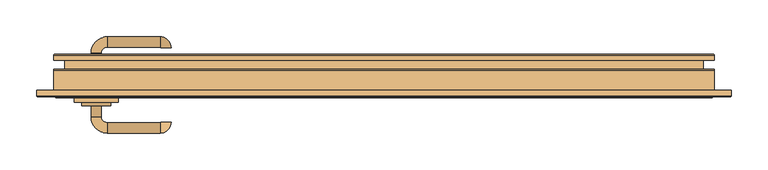
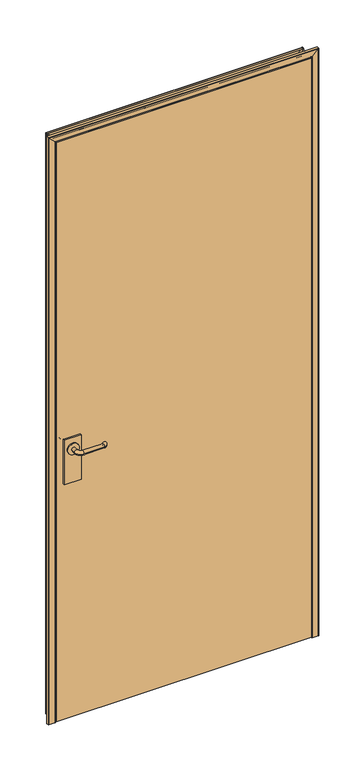
"""IFC4 building model written with IfcOpenShell, lengths in millimetres: door geometry, Porta Simples de Abrir : 90x210cm - Aduela Metálica de Canto."""

from ifc_helpers import new_model, si_unit, point, frame, frame_2d, origin, place, context, project, spatial, polyline, circle_curve, ellipse_curve, trimmed, segment, composite_curve, outline, extrude, source, transform, mapped, element, save
from ifc_brep_helpers import plane_surface, cylinder_surface, revolved_surface, advanced_brep


def door_e47fb599(model_context):
    return source(origin(), model_context, "Body", "SolidModel", [
        extrude(outline(composite_curve([segment(trimmed(circle_curve(frame_2d((1050.0, -392.0)), 20.0), [point((1050.0, -412.0))], [point((1050.0, -372.0))], False, "CARTESIAN"), True, "CONTINUOUS"), segment(trimmed(circle_curve(frame_2d((1050.0, -392.0)), 20.0), [point((1050.0, -372.0))], [point((1050.0, -412.0))], False, "CARTESIAN"), True, "CONTINUOUS")], self_intersect=False)), frame((0.0, -54.6, 0.0), z_axis=(0.0, 1.0, 0.0), x_axis=(0.0, 0.0, 1.0)), (0.0, 0.0, 1.0), 4.5929895),
        advanced_brep(
        [(-385.0, -50.0070105, 1050.0), (-399.0, -50.0070105, 1050.0), (-385.0, -34.6, 1050.0), (-399.0, -34.6, 1050.0), (-377.0, -12.6, 1050.0), (-377.0, -26.6, 1050.0), (-305.0, -26.6, 1050.0), (-305.0, -12.6, 1050.0), (-304.0, -27.6, 1050.0), (-290.0, -27.6, 1050.0)],
        [
            (0, 1, circle_curve(frame((-392.0, -50.0070105, 1050.0), z_axis=(0.0, -1.0, 0.0), x_axis=(-1.0, 0.0, 0.0)), 7.0)),
            (1, 0, circle_curve(frame((-392.0, -50.0070105, 1050.0), z_axis=(0.0, -1.0, 0.0), x_axis=(-1.0, 0.0, 0.0)), 7.0)),
            (0, 2),
            (2, 3, circle_curve(frame((-392.0, -34.6, 1050.0), z_axis=(0.0, -1.0, 0.0), x_axis=(-1.0, 0.0, 0.0)), 7.0)),
            (3, 1),
            (3, 2, circle_curve(frame((-392.0, -34.6, 1050.0), z_axis=(0.0, -1.0, 0.0), x_axis=(-1.0, 0.0, 0.0)), 7.0)),
            (4, 3, circle_curve(frame((-377.0, -34.6, 1050.0), z_axis=(0.0, 0.0, 1.0), x_axis=(-1.0, 0.0, 0.0)), 22.0)),
            (2, 5, circle_curve(frame((-377.0, -34.6, 1050.0), z_axis=(0.0, 0.0, -1.0), x_axis=(-1.0, 0.0, 0.0)), 8.0)),
            (5, 4, circle_curve(frame((-377.0, -19.6, 1050.0), z_axis=(-1.0, 0.0, 0.0), x_axis=(0.0, 1.0, 0.0)), 7.0)),
            (4, 5, circle_curve(frame((-377.0, -19.6, 1050.0), z_axis=(-1.0, 0.0, 0.0), x_axis=(0.0, 1.0, 0.0)), 7.0)),
            (5, 6),
            (6, 7, circle_curve(frame((-305.0, -19.6, 1050.0), z_axis=(-1.0, 0.0, 0.0), x_axis=(0.0, 1.0, 0.0)), 7.0)),
            (7, 4),
            (7, 6, circle_curve(frame((-305.0, -19.6, 1050.0), z_axis=(-1.0, 0.0, 0.0), x_axis=(0.0, 1.0, 0.0)), 7.0)),
            (8, 9, circle_curve(frame((-297.0, -27.6, 1050.0), z_axis=(0.0, -1.0, 0.0), x_axis=(1.0, 0.0, 0.0)), 7.0)),
            (9, 8, circle_curve(frame((-297.0, -27.6, 1050.0), z_axis=(0.0, -1.0, 0.0), x_axis=(1.0, 0.0, 0.0)), 7.0)),
            (9, 7, circle_curve(frame((-305.0, -27.6, 1050.0), z_axis=(0.0, 0.0, 1.0), x_axis=(0.0, 1.0, 0.0)), 15.0)),
            (6, 8, circle_curve(frame((-305.0, -27.6, 1050.0), z_axis=(0.0, 0.0, -1.0), x_axis=(0.0, 1.0, 0.0)), 1.0)),
        ],
        [
            plane_surface(frame((-392.0, -50.0070105, 1050.0), z_axis=(0.0, -1.0, 0.0), x_axis=(0.0, 0.0, 1.0))),
            cylinder_surface(frame((-392.0, -50.0070105, 1050.0), z_axis=(0.0, -1.0, 0.0), x_axis=(-1.0, 0.0, 0.0)), 7.0),
            revolved_surface(trimmed(ellipse_curve(frame((-392.0, -34.6, 1050.0), z_axis=(0.0, -1.0, 0.0), x_axis=(-1.0, 0.0, 0.0)), 7.0, 7.0), [point((-385.0, -34.6, 1050.0))], [point((-399.0, -34.6, 1050.0))], True, "CARTESIAN"), (-377.0, -34.6, 1050.0), (0.0, 0.0, -1.0)),
            revolved_surface(trimmed(ellipse_curve(frame((-392.0, -34.6, 1050.0), z_axis=(0.0, -1.0, 0.0), x_axis=(-1.0, 0.0, 0.0)), 7.0, 7.0), [point((-399.0, -34.6, 1050.0))], [point((-385.0, -34.6, 1050.0))], True, "CARTESIAN"), (-377.0, -34.6, 1050.0), (0.0, 0.0, -1.0)),
            cylinder_surface(frame((-377.0, -19.6, 1050.0), z_axis=(-1.0, 0.0, 0.0), x_axis=(0.0, 1.0, 0.0)), 7.0),
            plane_surface(frame((-297.0, -27.6, 1050.0), z_axis=(0.0, -1.0, 0.0), x_axis=(0.0, 0.0, 1.0))),
            revolved_surface(trimmed(ellipse_curve(frame((-305.0, -19.6, 1050.0), z_axis=(-1.0, 0.0, 0.0), x_axis=(0.0, 1.0, 0.0)), 7.0, 7.0), [point((-305.0, -26.6, 1050.0))], [point((-305.0, -12.6, 1050.0))], True, "CARTESIAN"), (-305.0, -27.6, 1050.0), (0.0, 0.0, -1.0)),
            revolved_surface(trimmed(ellipse_curve(frame((-305.0, -19.6, 1050.0), z_axis=(-1.0, 0.0, 0.0), x_axis=(0.0, 1.0, 0.0)), 7.0, 7.0), [point((-305.0, -12.6, 1050.0))], [point((-305.0, -26.6, 1050.0))], True, "CARTESIAN"), (-305.0, -27.6, 1050.0), (0.0, 0.0, -1.0)),
        ],
        [
            (0, [[1, 2]]),
            (1, [[-1, 3, 4, 5]]),
            (1, [[-2, -5, 6, -3]]),
            (2, [[7, -4, 8, 9]]),
            (3, [[-8, -6, -7, 10]]),
            (4, [[-9, 11, 12, 13]]),
            (4, [[-10, -13, 14, -11]]),
            (5, [[15, 16]]),
            (6, [[17, -12, 18, -16]]),
            (7, [[-18, -14, -17, -15]]),
        ],
    ),
        extrude(outline(polyline([(-362.0, -60.6), (-422.0, -60.6), (-422.0, -54.6), (-362.0, -54.6), (-362.0, -60.6)])), frame((0.0, 0.0, 925.0), z_axis=(0.0, 0.0, 1.0), x_axis=(1.0, 0.0, 0.0)), (0.0, 0.0, 1.0), 165.0),
        extrude(outline(composite_curve([segment(trimmed(circle_curve(frame_2d((1050.0, -392.0)), 20.0), [point((1050.0, -412.0))], [point((1050.0, -372.0))], False, "CARTESIAN"), True, "CONTINUOUS"), segment(trimmed(circle_curve(frame_2d((1050.0, -392.0)), 20.0), [point((1050.0, -372.0))], [point((1050.0, -412.0))], False, "CARTESIAN"), True, "CONTINUOUS")], self_intersect=False)), frame((0.0, -106.1929895, 0.0), z_axis=(0.0, 1.0, 0.0), x_axis=(0.0, 0.0, 1.0)), (0.0, 0.0, 1.0), 4.5929895),
        advanced_brep(
        [(-385.0, -106.1929895, 1050.0), (-399.0, -106.1929895, 1050.0), (-399.0, -121.6, 1050.0), (-385.0, -121.6, 1050.0), (-377.0, -143.6, 1050.0), (-377.0, -129.6, 1050.0), (-305.0, -143.6, 1050.0), (-305.0, -129.6, 1050.0), (-304.0, -128.6, 1050.0), (-290.0, -128.6, 1050.0)],
        [
            (0, 1, circle_curve(frame((-392.0, -106.1929895, 1050.0), z_axis=(0.0, 1.0, 0.0), x_axis=(-1.0, 0.0, 0.0)), 7.0)),
            (1, 0, circle_curve(frame((-392.0, -106.1929895, 1050.0), z_axis=(0.0, 1.0, 0.0), x_axis=(-1.0, 0.0, 0.0)), 7.0)),
            (1, 2),
            (2, 3, circle_curve(frame((-392.0, -121.6, 1050.0), z_axis=(0.0, 1.0, 0.0), x_axis=(-1.0, 0.0, 0.0)), 7.0)),
            (3, 0),
            (3, 2, circle_curve(frame((-392.0, -121.6, 1050.0), z_axis=(0.0, 1.0, 0.0), x_axis=(-1.0, 0.0, 0.0)), 7.0)),
            (4, 5, circle_curve(frame((-377.0, -136.6, 1050.0), z_axis=(-1.0, 0.0, 0.0), x_axis=(0.0, -1.0, 0.0)), 7.0)),
            (5, 3, circle_curve(frame((-377.0, -121.6, 1050.0), z_axis=(0.0, 0.0, -1.0), x_axis=(-1.0, 0.0, 0.0)), 8.0)),
            (2, 4, circle_curve(frame((-377.0, -121.6, 1050.0), z_axis=(0.0, 0.0, 1.0), x_axis=(-1.0, 0.0, 0.0)), 22.0)),
            (5, 4, circle_curve(frame((-377.0, -136.6, 1050.0), z_axis=(-1.0, 0.0, 0.0), x_axis=(0.0, -1.0, 0.0)), 7.0)),
            (4, 6),
            (6, 7, circle_curve(frame((-305.0, -136.6, 1050.0), z_axis=(-1.0, 0.0, 0.0), x_axis=(0.0, -1.0, 0.0)), 7.0)),
            (7, 5),
            (7, 6, circle_curve(frame((-305.0, -136.6, 1050.0), z_axis=(-1.0, 0.0, 0.0), x_axis=(0.0, -1.0, 0.0)), 7.0)),
            (8, 9, circle_curve(frame((-297.0, -128.6, 1050.0), z_axis=(0.0, 1.0, 0.0), x_axis=(1.0, 0.0, 0.0)), 7.0)),
            (9, 8, circle_curve(frame((-297.0, -128.6, 1050.0), z_axis=(0.0, 1.0, 0.0), x_axis=(1.0, 0.0, 0.0)), 7.0)),
            (8, 7, circle_curve(frame((-305.0, -128.6, 1050.0), z_axis=(0.0, 0.0, -1.0), x_axis=(0.0, -1.0, 0.0)), 1.0)),
            (6, 9, circle_curve(frame((-305.0, -128.6, 1050.0), z_axis=(0.0, 0.0, 1.0), x_axis=(0.0, -1.0, 0.0)), 15.0)),
        ],
        [
            plane_surface(frame((-392.0, -106.1929895, 1050.0), z_axis=(0.0, 1.0, 0.0), x_axis=(0.0, 0.0, 1.0))),
            cylinder_surface(frame((-392.0, -106.1929895, 1050.0), z_axis=(0.0, 1.0, 0.0), x_axis=(-1.0, 0.0, 0.0)), 7.0),
            revolved_surface(trimmed(ellipse_curve(frame((-392.0, -121.6, 1050.0), z_axis=(0.0, -1.0, 0.0), x_axis=(-1.0, 0.0, 0.0)), 7.0, 7.0), [point((-385.0, -121.6, 1050.0))], [point((-399.0, -121.6, 1050.0))], True, "CARTESIAN"), (-377.0, -121.6, 1050.0), (0.0, 0.0, -1.0)),
            revolved_surface(trimmed(ellipse_curve(frame((-392.0, -121.6, 1050.0), z_axis=(0.0, -1.0, 0.0), x_axis=(-1.0, 0.0, 0.0)), 7.0, 7.0), [point((-399.0, -121.6, 1050.0))], [point((-385.0, -121.6, 1050.0))], True, "CARTESIAN"), (-377.0, -121.6, 1050.0), (0.0, 0.0, -1.0)),
            cylinder_surface(frame((-377.0, -136.6, 1050.0), z_axis=(-1.0, 0.0, 0.0), x_axis=(0.0, -1.0, 0.0)), 7.0),
            plane_surface(frame((-297.0, -128.6, 1050.0), z_axis=(0.0, 1.0, 0.0), x_axis=(0.0, 0.0, 1.0))),
            revolved_surface(trimmed(ellipse_curve(frame((-305.0, -136.6, 1050.0), z_axis=(1.0, 0.0, 0.0), x_axis=(0.0, -1.0, 0.0)), 7.0, 7.0), [point((-305.0, -129.6, 1050.0))], [point((-305.0, -143.6, 1050.0))], True, "CARTESIAN"), (-305.0, -128.6, 1050.0), (0.0, 0.0, -1.0)),
            revolved_surface(trimmed(ellipse_curve(frame((-305.0, -136.6, 1050.0), z_axis=(1.0, 0.0, 0.0), x_axis=(0.0, -1.0, 0.0)), 7.0, 7.0), [point((-305.0, -143.6, 1050.0))], [point((-305.0, -129.6, 1050.0))], True, "CARTESIAN"), (-305.0, -128.6, 1050.0), (0.0, 0.0, -1.0)),
        ],
        [
            (0, [[1, 2]]),
            (1, [[3, 4, 5, -2]]),
            (1, [[-5, 6, -3, -1]]),
            (2, [[7, 8, -4, 9]]),
            (3, [[10, -9, -6, -8]]),
            (4, [[11, 12, 13, -7]]),
            (4, [[-13, 14, -11, -10]]),
            (5, [[15, 16]]),
            (6, [[-15, 17, -12, 18]]),
            (7, [[-16, -18, -14, -17]]),
        ],
    ),
        extrude(outline(polyline([(-362.0, -95.6), (-362.0, -101.6), (-422.0, -101.6), (-422.0, -95.6), (-362.0, -95.6)])), frame((0.0, 0.0, 925.0), z_axis=(0.0, 0.0, 1.0), x_axis=(1.0, 0.0, 0.0)), (0.0, 0.0, 1.0), 165.0),
        extrude(outline(polyline([(447.0, -60.6), (447.0, -95.6), (-447.0, -95.6), (-447.0, -60.6), (447.0, -60.6)])), frame((0.0, 0.0, 53.0), z_axis=(0.0, 0.0, 1.0), x_axis=(1.0, 0.0, 0.0)), (0.0, 0.0, 1.0), 2143.0),
        advanced_brep(
        [(-435.5, -36.6, 50.0), (-434.0, -38.1, 50.0), (-434.0, -56.1, 50.0), (-435.5, -57.6, 50.0), (-448.55, -57.6, 50.0), (-449.05, -58.1, 50.0), (-449.05, -93.1, 50.0), (-450.55, -94.6, 50.0), (-471.55, -94.6, 50.0), (-473.05, -93.1, 50.0), (-473.05, -85.6, 50.0), (-472.05, -85.6, 50.0), (-472.05, -93.1, 50.0), (-471.55, -93.6, 50.0), (-450.55, -93.6, 50.0), (-450.05, -93.1, 50.0), (-450.05, -58.1, 50.0), (-448.55, -56.6, 50.0), (-435.5, -56.6, 50.0), (-435.0, -56.1, 50.0), (-435.0, -38.1, 50.0), (-435.5, -37.6, 50.0), (-448.5, -37.6, 50.0), (-449.0, -38.1, 50.0), (-449.0, -44.6, 50.0), (-450.0, -44.6, 50.0), (-450.0, -38.1, 50.0), (-448.5, -36.6, 50.0), (-448.5, -36.6, 2198.5), (-435.5, -36.6, 2185.5), (-450.0, -38.1, 2200.0), (-450.0, -44.6, 2200.0), (-449.0, -44.6, 2199.0), (-449.0, -38.1, 2199.0), (-448.5, -37.6, 2198.5), (-435.5, -37.6, 2185.5), (-435.0, -38.1, 2185.0), (-435.0, -56.1, 2185.0), (-435.5, -56.6, 2185.5), (-448.55, -56.6, 2198.55), (-450.05, -58.1, 2200.05), (-450.05, -93.1, 2200.05), (-450.55, -93.6, 2200.55), (-471.55, -93.6, 2221.55), (-472.05, -93.1, 2222.05), (-472.05, -85.6, 2222.05), (-473.05, -85.6, 2223.05), (-473.05, -93.1, 2223.05), (-471.55, -94.6, 2221.55), (-450.55, -94.6, 2200.55), (-449.05, -93.1, 2199.05), (-449.05, -58.1, 2199.05), (-448.55, -57.6, 2198.55), (-435.5, -57.6, 2185.5), (-434.0, -56.1, 2184.0), (-434.0, -38.1, 2184.0), (435.5, -36.6, 50.0), (448.5, -36.6, 50.0), (450.0, -38.1, 50.0), (450.0, -44.6, 50.0), (449.0, -44.6, 50.0), (449.0, -38.1, 50.0), (448.5, -37.6, 50.0), (435.5, -37.6, 50.0), (435.0, -38.1, 50.0), (435.0, -56.1, 50.0), (435.5, -56.6, 50.0), (448.55, -56.6, 50.0), (450.05, -58.1, 50.0), (450.05, -93.1, 50.0), (450.55, -93.6, 50.0), (471.55, -93.6, 50.0), (472.05, -93.1, 50.0), (472.05, -85.6, 50.0), (473.05, -85.6, 50.0), (473.05, -93.1, 50.0), (471.55, -94.6, 50.0), (450.55, -94.6, 50.0), (449.05, -93.1, 50.0), (449.05, -58.1, 50.0), (448.55, -57.6, 50.0), (435.5, -57.6, 50.0), (434.0, -56.1, 50.0), (434.0, -38.1, 50.0), (435.5, -36.6, 2185.5), (434.0, -38.1, 2184.0), (434.0, -56.1, 2184.0), (435.5, -57.6, 2185.5), (448.55, -57.6, 2198.55), (449.05, -58.1, 2199.05), (449.05, -93.1, 2199.05), (450.55, -94.6, 2200.55), (471.55, -94.6, 2221.55), (473.05, -93.1, 2223.05), (473.05, -85.6, 2223.05), (472.05, -85.6, 2222.05), (472.05, -93.1, 2222.05), (471.55, -93.6, 2221.55), (450.55, -93.6, 2200.55), (450.05, -93.1, 2200.05), (450.05, -58.1, 2200.05), (448.55, -56.6, 2198.55), (435.5, -56.6, 2185.5), (435.0, -56.1, 2185.0), (435.0, -38.1, 2185.0), (435.5, -37.6, 2185.5), (448.5, -37.6, 2198.5), (449.0, -38.1, 2199.0), (449.0, -44.6, 2199.0), (450.0, -44.6, 2200.0), (450.0, -38.1, 2200.0), (448.5, -36.6, 2198.5)],
        [
            (0, 1, circle_curve(frame((-435.5, -38.1, 50.0), z_axis=(0.0, 0.0, -1.0), x_axis=(1.0, 0.0, 0.0)), 1.5)),
            (1, 2),
            (2, 3, circle_curve(frame((-435.5, -56.1, 50.0), z_axis=(0.0, 0.0, -1.0), x_axis=(1.0, 0.0, 0.0)), 1.5)),
            (3, 4),
            (4, 5, circle_curve(frame((-448.55, -58.1, 50.0), z_axis=(0.0, 0.0, 1.0), x_axis=(1.0, 0.0, 0.0)), 0.5)),
            (5, 6),
            (6, 7, circle_curve(frame((-450.55, -93.1, 50.0), z_axis=(0.0, 0.0, -1.0), x_axis=(1.0, 0.0, 0.0)), 1.5)),
            (7, 8),
            (8, 9, circle_curve(frame((-471.55, -93.1, 50.0), z_axis=(0.0, 0.0, -1.0), x_axis=(1.0, 0.0, 0.0)), 1.5)),
            (9, 10),
            (10, 11),
            (11, 12),
            (12, 13, circle_curve(frame((-471.55, -93.1, 50.0), z_axis=(0.0, 0.0, 1.0), x_axis=(1.0, 0.0, 0.0)), 0.5)),
            (13, 14),
            (14, 15, circle_curve(frame((-450.55, -93.1, 50.0), z_axis=(0.0, 0.0, 1.0), x_axis=(1.0, 0.0, 0.0)), 0.5)),
            (15, 16),
            (16, 17, circle_curve(frame((-448.55, -58.1, 50.0), z_axis=(0.0, 0.0, -1.0), x_axis=(1.0, 0.0, 0.0)), 1.5)),
            (17, 18),
            (18, 19, circle_curve(frame((-435.5, -56.1, 50.0), z_axis=(0.0, 0.0, 1.0), x_axis=(1.0, 0.0, 0.0)), 0.5)),
            (19, 20),
            (20, 21, circle_curve(frame((-435.5, -38.1, 50.0), z_axis=(0.0, 0.0, 1.0), x_axis=(1.0, 0.0, 0.0)), 0.5)),
            (21, 22),
            (22, 23, circle_curve(frame((-448.5, -38.1, 50.0), z_axis=(0.0, 0.0, 1.0), x_axis=(1.0, 0.0, 0.0)), 0.5)),
            (23, 24),
            (24, 25),
            (25, 26),
            (26, 27, circle_curve(frame((-448.5, -38.1, 50.0), z_axis=(0.0, 0.0, -1.0), x_axis=(1.0, 0.0, 0.0)), 1.5)),
            (27, 0),
            (27, 28),
            (28, 29),
            (29, 0),
            (26, 30),
            (30, 28, ellipse_curve(frame((-448.5, -38.1, 2198.5), z_axis=(-0.7071067811865475, 0.0, -0.7071067811865475), x_axis=(0.7071067811865474, 0.0, -0.7071067811865476)), 2.1213203, 1.5)),
            (25, 31),
            (31, 30),
            (24, 32),
            (32, 31),
            (23, 33),
            (33, 32),
            (22, 34),
            (34, 33, ellipse_curve(frame((-448.5, -38.1, 2198.5), z_axis=(0.7071067811865475, 0.0, 0.7071067811865475), x_axis=(-0.7071067811865474, 0.0, 0.7071067811865476)), 0.7071068, 0.5)),
            (21, 35),
            (35, 34),
            (20, 36),
            (36, 35, ellipse_curve(frame((-435.5, -38.1, 2185.5), z_axis=(0.7071067811865475, 0.0, 0.7071067811865475), x_axis=(-0.7071067811865474, 0.0, 0.7071067811865476)), 0.7071068, 0.5)),
            (19, 37),
            (37, 36),
            (18, 38),
            (38, 37, ellipse_curve(frame((-435.5, -56.1, 2185.5), z_axis=(0.7071067811865475, 0.0, 0.7071067811865475), x_axis=(-0.7071067811865474, 0.0, 0.7071067811865476)), 0.7071068, 0.5)),
            (17, 39),
            (39, 38),
            (16, 40),
            (40, 39, ellipse_curve(frame((-448.55, -58.1, 2198.55), z_axis=(-0.7071067811865475, 0.0, -0.7071067811865475), x_axis=(0.7071067811865474, 0.0, -0.7071067811865476)), 2.1213203, 1.5)),
            (15, 41),
            (41, 40),
            (14, 42),
            (42, 41, ellipse_curve(frame((-450.55, -93.1, 2200.55), z_axis=(0.7071067811865475, 0.0, 0.7071067811865475), x_axis=(-0.7071067811865474, 0.0, 0.7071067811865476)), 0.7071068, 0.5)),
            (13, 43),
            (43, 42),
            (12, 44),
            (44, 43, ellipse_curve(frame((-471.55, -93.1, 2221.55), z_axis=(0.7071067811865475, 0.0, 0.7071067811865475), x_axis=(-0.7071067811865474, 0.0, 0.7071067811865476)), 0.7071068, 0.5)),
            (11, 45),
            (45, 44),
            (10, 46),
            (46, 45),
            (9, 47),
            (47, 46),
            (8, 48),
            (48, 47, ellipse_curve(frame((-471.55, -93.1, 2221.55), z_axis=(-0.7071067811865475, 0.0, -0.7071067811865475), x_axis=(0.7071067811865474, 0.0, -0.7071067811865476)), 2.1213203, 1.5)),
            (7, 49),
            (49, 48),
            (6, 50),
            (50, 49, ellipse_curve(frame((-450.55, -93.1, 2200.55), z_axis=(-0.7071067811865475, 0.0, -0.7071067811865475), x_axis=(0.7071067811865474, 0.0, -0.7071067811865476)), 2.1213203, 1.5)),
            (5, 51),
            (51, 50),
            (4, 52),
            (52, 51, ellipse_curve(frame((-448.55, -58.1, 2198.55), z_axis=(0.7071067811865475, 0.0, 0.7071067811865475), x_axis=(-0.7071067811865474, 0.0, 0.7071067811865476)), 0.7071068, 0.5)),
            (3, 53),
            (53, 52),
            (2, 54),
            (54, 53, ellipse_curve(frame((-435.5, -56.1, 2185.5), z_axis=(-0.7071067811865475, 0.0, -0.7071067811865475), x_axis=(0.7071067811865474, 0.0, -0.7071067811865476)), 2.1213203, 1.5)),
            (1, 55),
            (55, 54),
            (29, 55, ellipse_curve(frame((-435.5, -38.1, 2185.5), z_axis=(-0.7071067811865475, 0.0, -0.7071067811865475), x_axis=(0.7071067811865474, 0.0, -0.7071067811865476)), 2.1213203, 1.5)),
            (56, 57),
            (57, 58, circle_curve(frame((448.5, -38.1, 50.0), z_axis=(0.0, 0.0, -1.0), x_axis=(-1.0, 0.0, 0.0)), 1.5)),
            (58, 59),
            (59, 60),
            (60, 61),
            (61, 62, circle_curve(frame((448.5, -38.1, 50.0), z_axis=(0.0, 0.0, 1.0), x_axis=(-1.0, 0.0, 0.0)), 0.5)),
            (62, 63),
            (63, 64, circle_curve(frame((435.5, -38.1, 50.0), z_axis=(0.0, 0.0, 1.0), x_axis=(-1.0, 0.0, 0.0)), 0.5)),
            (64, 65),
            (65, 66, circle_curve(frame((435.5, -56.1, 50.0), z_axis=(0.0, 0.0, 1.0), x_axis=(-1.0, 0.0, 0.0)), 0.5)),
            (66, 67),
            (67, 68, circle_curve(frame((448.55, -58.1, 50.0), z_axis=(0.0, 0.0, -1.0), x_axis=(-1.0, 0.0, 0.0)), 1.5)),
            (68, 69),
            (69, 70, circle_curve(frame((450.55, -93.1, 50.0), z_axis=(0.0, 0.0, 1.0), x_axis=(-1.0, 0.0, 0.0)), 0.5)),
            (70, 71),
            (71, 72, circle_curve(frame((471.55, -93.1, 50.0), z_axis=(0.0, 0.0, 1.0), x_axis=(-1.0, 0.0, 0.0)), 0.5)),
            (72, 73),
            (73, 74),
            (74, 75),
            (75, 76, circle_curve(frame((471.55, -93.1, 50.0), z_axis=(0.0, 0.0, -1.0), x_axis=(-1.0, 0.0, 0.0)), 1.5)),
            (76, 77),
            (77, 78, circle_curve(frame((450.55, -93.1, 50.0), z_axis=(0.0, 0.0, -1.0), x_axis=(-1.0, 0.0, 0.0)), 1.5)),
            (78, 79),
            (79, 80, circle_curve(frame((448.55, -58.1, 50.0), z_axis=(0.0, 0.0, 1.0), x_axis=(-1.0, 0.0, 0.0)), 0.5)),
            (80, 81),
            (81, 82, circle_curve(frame((435.5, -56.1, 50.0), z_axis=(0.0, 0.0, -1.0), x_axis=(-1.0, 0.0, 0.0)), 1.5)),
            (82, 83),
            (83, 56, circle_curve(frame((435.5, -38.1, 50.0), z_axis=(0.0, 0.0, -1.0), x_axis=(-1.0, 0.0, 0.0)), 1.5)),
            (84, 56),
            (83, 85),
            (85, 84, ellipse_curve(frame((435.5, -38.1, 2185.5), z_axis=(0.7071067811865475, 0.0, -0.7071067811865475), x_axis=(0.7071067811865474, 0.0, 0.7071067811865476)), 2.1213203, 1.5)),
            (82, 86),
            (86, 85),
            (81, 87),
            (87, 86, ellipse_curve(frame((435.5, -56.1, 2185.5), z_axis=(0.7071067811865475, 0.0, -0.7071067811865475), x_axis=(0.7071067811865474, 0.0, 0.7071067811865476)), 2.1213203, 1.5)),
            (80, 88),
            (88, 87),
            (79, 89),
            (89, 88, ellipse_curve(frame((448.55, -58.1, 2198.55), z_axis=(-0.7071067811865475, 0.0, 0.7071067811865475), x_axis=(-0.7071067811865474, 0.0, -0.7071067811865476)), 0.7071068, 0.5)),
            (78, 90),
            (90, 89),
            (77, 91),
            (91, 90, ellipse_curve(frame((450.55, -93.1, 2200.55), z_axis=(0.7071067811865475, 0.0, -0.7071067811865475), x_axis=(0.7071067811865474, 0.0, 0.7071067811865476)), 2.1213203, 1.5)),
            (76, 92),
            (92, 91),
            (75, 93),
            (93, 92, ellipse_curve(frame((471.55, -93.1, 2221.55), z_axis=(0.7071067811865475, 0.0, -0.7071067811865475), x_axis=(0.7071067811865474, 0.0, 0.7071067811865476)), 2.1213203, 1.5)),
            (74, 94),
            (94, 93),
            (73, 95),
            (95, 94),
            (72, 96),
            (96, 95),
            (71, 97),
            (97, 96, ellipse_curve(frame((471.55, -93.1, 2221.55), z_axis=(-0.7071067811865475, 0.0, 0.7071067811865475), x_axis=(-0.7071067811865474, 0.0, -0.7071067811865476)), 0.7071068, 0.5)),
            (70, 98),
            (98, 97),
            (69, 99),
            (99, 98, ellipse_curve(frame((450.55, -93.1, 2200.55), z_axis=(-0.7071067811865475, 0.0, 0.7071067811865475), x_axis=(-0.7071067811865474, 0.0, -0.7071067811865476)), 0.7071068, 0.5)),
            (68, 100),
            (100, 99),
            (67, 101),
            (101, 100, ellipse_curve(frame((448.55, -58.1, 2198.55), z_axis=(0.7071067811865475, 0.0, -0.7071067811865475), x_axis=(0.7071067811865474, 0.0, 0.7071067811865476)), 2.1213203, 1.5)),
            (66, 102),
            (102, 101),
            (65, 103),
            (103, 102, ellipse_curve(frame((435.5, -56.1, 2185.5), z_axis=(-0.7071067811865475, 0.0, 0.7071067811865475), x_axis=(-0.7071067811865474, 0.0, -0.7071067811865476)), 0.7071068, 0.5)),
            (64, 104),
            (104, 103),
            (63, 105),
            (105, 104, ellipse_curve(frame((435.5, -38.1, 2185.5), z_axis=(-0.7071067811865475, 0.0, 0.7071067811865475), x_axis=(-0.7071067811865474, 0.0, -0.7071067811865476)), 0.7071068, 0.5)),
            (62, 106),
            (106, 105),
            (61, 107),
            (107, 106, ellipse_curve(frame((448.5, -38.1, 2198.5), z_axis=(-0.7071067811865475, 0.0, 0.7071067811865475), x_axis=(-0.7071067811865474, 0.0, -0.7071067811865476)), 0.7071068, 0.5)),
            (60, 108),
            (108, 107),
            (59, 109),
            (109, 108),
            (58, 110),
            (110, 109),
            (57, 111),
            (111, 110, ellipse_curve(frame((448.5, -38.1, 2198.5), z_axis=(0.7071067811865475, 0.0, -0.7071067811865475), x_axis=(0.7071067811865474, 0.0, 0.7071067811865476)), 2.1213203, 1.5)),
            (84, 111),
            (28, 111),
            (84, 29),
            (30, 110),
            (31, 109),
            (32, 108),
            (33, 107),
            (34, 106),
            (35, 105),
            (36, 104),
            (37, 103),
            (38, 102),
            (39, 101),
            (40, 100),
            (41, 99),
            (42, 98),
            (43, 97),
            (44, 96),
            (45, 95),
            (46, 94),
            (47, 93),
            (48, 92),
            (49, 91),
            (50, 90),
            (51, 89),
            (52, 88),
            (53, 87),
            (54, 86),
            (55, 85),
        ],
        [
            plane_surface(frame((-450.0, -34.4996086, 50.0), z_axis=(0.0, 0.0, -1.0), x_axis=(1.0, 0.0, 0.0))),
            plane_surface(frame((-435.5, -36.6, 50.0), z_axis=(0.0, 1.0, 0.0), x_axis=(0.0, 0.0, 1.0))),
            cylinder_surface(frame((-448.5, -38.1, 50.0), z_axis=(0.0, 0.0, -1.0), x_axis=(1.0, 0.0, 0.0)), 1.5),
            plane_surface(frame((-450.0, -38.1, 50.0), z_axis=(-1.0, 0.0, 0.0), x_axis=(0.0, 0.0, 1.0))),
            plane_surface(frame((-450.0, -44.6, 50.0), z_axis=(0.0, -1.0, 0.0), x_axis=(0.0, 0.0, 1.0))),
            plane_surface(frame((-449.0, -44.6, 50.0), z_axis=(1.0, 0.0, 0.0), x_axis=(0.0, 0.0, 1.0))),
            revolved_surface(polyline([(-448.0, -38.1, 2199.000000013303), (-448.0, -38.1, 50.0)]), (-448.5, -38.1, 50.0), (0.0, 0.0, 1.0)),
            plane_surface(frame((-448.5, -37.6, 50.0), z_axis=(0.0, -1.0, 0.0), x_axis=(0.0, 0.0, 1.0))),
            revolved_surface(polyline([(-435.0, -38.1, 2186.000000013303), (-435.0, -38.1, 50.0)]), (-435.5, -38.1, 50.0), (0.0, 0.0, 1.0)),
            plane_surface(frame((-435.0, -38.1, 50.0), z_axis=(-1.0, 0.0, 0.0), x_axis=(0.0, 0.0, 1.0))),
            revolved_surface(polyline([(-435.0, -56.1, 2186.000000013303), (-435.0, -56.1, 50.0)]), (-435.5, -56.1, 50.0), (0.0, 0.0, 1.0)),
            plane_surface(frame((-435.5, -56.6, 50.0), z_axis=(0.0, 1.0, 0.0), x_axis=(0.0, 0.0, 1.0))),
            cylinder_surface(frame((-448.55, -58.1, 50.0), z_axis=(0.0, 0.0, -1.0), x_axis=(1.0, 0.0, 0.0)), 1.5),
            plane_surface(frame((-450.05, -58.1, 50.0), z_axis=(-1.0, 0.0, 0.0), x_axis=(0.0, 0.0, 1.0))),
            revolved_surface(polyline([(-450.05, -93.1, 2201.0500000133034), (-450.05, -93.1, 50.0)]), (-450.55, -93.1, 50.0), (0.0, 0.0, 1.0)),
            plane_surface(frame((-450.55, -93.6, 50.0), z_axis=(0.0, 1.0, 0.0), x_axis=(0.0, 0.0, 1.0))),
            revolved_surface(polyline([(-471.05, -93.1, 2222.0500000133034), (-471.05, -93.1, 50.0)]), (-471.55, -93.1, 50.0), (0.0, 0.0, 1.0)),
            plane_surface(frame((-472.05, -93.1, 50.0), z_axis=(1.0, 0.0, 0.0), x_axis=(0.0, 0.0, 1.0))),
            plane_surface(frame((-472.05, -85.6, 50.0), z_axis=(0.0, 1.0, 0.0), x_axis=(0.0, 0.0, 1.0))),
            plane_surface(frame((-473.05, -85.6, 50.0), z_axis=(-1.0, 0.0, 0.0), x_axis=(0.0, 0.0, 1.0))),
            cylinder_surface(frame((-471.55, -93.1, 50.0), z_axis=(0.0, 0.0, -1.0), x_axis=(1.0, 0.0, 0.0)), 1.5),
            plane_surface(frame((-471.55, -94.6, 50.0), z_axis=(0.0, -1.0, 0.0), x_axis=(0.0, 0.0, 1.0))),
            cylinder_surface(frame((-450.55, -93.1, 50.0), z_axis=(0.0, 0.0, -1.0), x_axis=(1.0, 0.0, 0.0)), 1.5),
            plane_surface(frame((-449.05, -93.1, 50.0), z_axis=(1.0, 0.0, 0.0), x_axis=(0.0, 0.0, 1.0))),
            revolved_surface(polyline([(-448.05, -58.1, 2199.0500000133034), (-448.05, -58.1, 50.0)]), (-448.55, -58.1, 50.0), (0.0, 0.0, 1.0)),
            plane_surface(frame((-448.55, -57.6, 50.0), z_axis=(0.0, -1.0, 0.0), x_axis=(0.0, 0.0, 1.0))),
            cylinder_surface(frame((-435.5, -56.1, 50.0), z_axis=(0.0, 0.0, -1.0), x_axis=(1.0, 0.0, 0.0)), 1.5),
            plane_surface(frame((-434.0, -56.1, 50.0), z_axis=(1.0, 0.0, 0.0), x_axis=(0.0, 0.0, 1.0))),
            cylinder_surface(frame((-435.5, -38.1, 50.0), z_axis=(0.0, 0.0, -1.0), x_axis=(1.0, 0.0, 0.0)), 1.5),
            plane_surface(frame((450.0, -34.4996086, 50.0), z_axis=(0.0, 0.0, -1.0), x_axis=(-1.0, 0.0, 0.0))),
            cylinder_surface(frame((435.5, -38.1, 2200.0), z_axis=(0.0, 0.0, 1.0), x_axis=(-1.0, 0.0, 0.0)), 1.5),
            plane_surface(frame((434.0, -56.1, 2184.0), z_axis=(-1.0, 0.0, 0.0), x_axis=(0.0, 0.0, -1.0))),
            cylinder_surface(frame((435.5, -56.1, 2200.0), z_axis=(0.0, 0.0, 1.0), x_axis=(-1.0, 0.0, 0.0)), 1.5),
            plane_surface(frame((448.55, -57.6, 2198.55), z_axis=(0.0, -1.0, 0.0), x_axis=(0.0, 0.0, -1.0))),
            revolved_surface(polyline([(448.05, -58.1, 50.0), (448.05, -58.1, 2199.0500000133034)]), (448.55, -58.1, 2200.0), (0.0, 0.0, -1.0)),
            plane_surface(frame((449.05, -93.1, 2199.05), z_axis=(-1.0, 0.0, 0.0), x_axis=(0.0, 0.0, -1.0))),
            cylinder_surface(frame((450.55, -93.1, 2200.0), z_axis=(0.0, 0.0, 1.0), x_axis=(-1.0, 0.0, 0.0)), 1.5),
            plane_surface(frame((471.55, -94.6, 2221.55), z_axis=(0.0, -1.0, 0.0), x_axis=(0.0, 0.0, -1.0))),
            cylinder_surface(frame((471.55, -93.1, 2200.0), z_axis=(0.0, 0.0, 1.0), x_axis=(-1.0, 0.0, 0.0)), 1.5),
            plane_surface(frame((473.05, -85.6, 2223.05), z_axis=(1.0, 0.0, 0.0), x_axis=(0.0, 0.0, -1.0))),
            plane_surface(frame((472.05, -85.6, 2222.05), z_axis=(0.0, 1.0, 0.0), x_axis=(0.0, 0.0, -1.0))),
            plane_surface(frame((472.05, -93.1, 2222.05), z_axis=(-1.0, 0.0, 0.0), x_axis=(0.0, 0.0, -1.0))),
            revolved_surface(polyline([(471.05, -93.1, 50.0), (471.05, -93.1, 2222.0500000133034)]), (471.55, -93.1, 2200.0), (0.0, 0.0, -1.0)),
            plane_surface(frame((450.55, -93.6, 2200.55), z_axis=(0.0, 1.0, 0.0), x_axis=(0.0, 0.0, -1.0))),
            revolved_surface(polyline([(450.05, -93.1, 50.0), (450.05, -93.1, 2201.0500000133034)]), (450.55, -93.1, 2200.0), (0.0, 0.0, -1.0)),
            plane_surface(frame((450.05, -58.1, 2200.05), z_axis=(1.0, 0.0, 0.0), x_axis=(0.0, 0.0, -1.0))),
            cylinder_surface(frame((448.55, -58.1, 2200.0), z_axis=(0.0, 0.0, 1.0), x_axis=(-1.0, 0.0, 0.0)), 1.5),
            plane_surface(frame((435.5, -56.6, 2185.5), z_axis=(0.0, 1.0, 0.0), x_axis=(0.0, 0.0, -1.0))),
            revolved_surface(polyline([(435.0, -56.1, 50.0), (435.0, -56.1, 2186.000000013303)]), (435.5, -56.1, 2200.0), (0.0, 0.0, -1.0)),
            plane_surface(frame((435.0, -38.1, 2185.0), z_axis=(1.0, 0.0, 0.0), x_axis=(0.0, 0.0, -1.0))),
            revolved_surface(polyline([(435.0, -38.1, 50.0), (435.0, -38.1, 2186.000000013303)]), (435.5, -38.1, 2200.0), (0.0, 0.0, -1.0)),
            plane_surface(frame((448.5, -37.6, 2198.5), z_axis=(0.0, -1.0, 0.0), x_axis=(0.0, 0.0, -1.0))),
            revolved_surface(polyline([(448.0, -38.1, 50.0), (448.0, -38.1, 2199.000000013303)]), (448.5, -38.1, 2200.0), (0.0, 0.0, -1.0)),
            plane_surface(frame((449.0, -44.6, 2199.0), z_axis=(-1.0, 0.0, 0.0), x_axis=(0.0, 0.0, -1.0))),
            plane_surface(frame((450.0, -44.6, 2200.0), z_axis=(0.0, -1.0, 0.0), x_axis=(0.0, 0.0, -1.0))),
            plane_surface(frame((450.0, -38.1, 2200.0), z_axis=(1.0, 0.0, 0.0), x_axis=(0.0, 0.0, -1.0))),
            cylinder_surface(frame((448.5, -38.1, 2200.0), z_axis=(0.0, 0.0, 1.0), x_axis=(-1.0, 0.0, 0.0)), 1.5),
            plane_surface(frame((435.5, -36.6, 2185.5), z_axis=(0.0, 1.0, 0.0), x_axis=(0.0, 0.0, -1.0))),
            plane_surface(frame((-435.5, -36.6, 2185.5), z_axis=(0.0, 1.0, 0.0), x_axis=(1.0, 0.0, 0.0))),
            cylinder_surface(frame((-450.0, -38.1, 2198.5), z_axis=(-1.0, 0.0, 0.0), x_axis=(0.0, 0.0, -1.0)), 1.5),
            plane_surface(frame((-450.0, -38.1, 2200.0), z_axis=(0.0, 0.0, 1.0), x_axis=(1.0, 0.0, 0.0))),
            plane_surface(frame((-450.0, -44.6, 2200.0), z_axis=(0.0, -1.0, 0.0), x_axis=(1.0, 0.0, 0.0))),
            plane_surface(frame((-449.0, -44.6, 2199.0), z_axis=(0.0, 0.0, -1.0), x_axis=(1.0, 0.0, 0.0))),
            revolved_surface(polyline([(449.00000001330307, -38.1, 2198.0), (-449.0000000133031, -38.1, 2198.0)]), (-450.0, -38.1, 2198.5), (1.0, 0.0, 0.0)),
            plane_surface(frame((-448.5, -37.6, 2198.5), z_axis=(0.0, -1.0, 0.0), x_axis=(1.0, 0.0, 0.0))),
            revolved_surface(polyline([(436.00000001330307, -38.1, 2185.0), (-436.0000000133031, -38.1, 2185.0)]), (-450.0, -38.1, 2185.5), (1.0, 0.0, 0.0)),
            plane_surface(frame((-435.0, -38.1, 2185.0), z_axis=(0.0, 0.0, 1.0), x_axis=(1.0, 0.0, 0.0))),
            revolved_surface(polyline([(436.00000001330307, -56.1, 2185.0), (-436.0000000133031, -56.1, 2185.0)]), (-450.0, -56.1, 2185.5), (1.0, 0.0, 0.0)),
            plane_surface(frame((-435.5, -56.6, 2185.5), z_axis=(0.0, 1.0, 0.0), x_axis=(1.0, 0.0, 0.0))),
            cylinder_surface(frame((-450.0, -58.1, 2198.55), z_axis=(-1.0, 0.0, 0.0), x_axis=(0.0, 0.0, -1.0)), 1.5),
            plane_surface(frame((-450.05, -58.1, 2200.05), z_axis=(0.0, 0.0, 1.0), x_axis=(1.0, 0.0, 0.0))),
            revolved_surface(polyline([(451.050000013303, -93.1, 2200.05), (-451.05000001330313, -93.1, 2200.05)]), (-450.0, -93.1, 2200.55), (1.0, 0.0, 0.0)),
            plane_surface(frame((-450.55, -93.6, 2200.55), z_axis=(0.0, 1.0, 0.0), x_axis=(1.0, 0.0, 0.0))),
            revolved_surface(polyline([(472.050000013303, -93.1, 2221.05), (-472.05000001330313, -93.1, 2221.05)]), (-450.0, -93.1, 2221.55), (1.0, 0.0, 0.0)),
            plane_surface(frame((-472.05, -93.1, 2222.05), z_axis=(0.0, 0.0, -1.0), x_axis=(1.0, 0.0, 0.0))),
            plane_surface(frame((-472.05, -85.6, 2222.05), z_axis=(0.0, 1.0, 0.0), x_axis=(1.0, 0.0, 0.0))),
            plane_surface(frame((-473.05, -85.6, 2223.05), z_axis=(0.0, 0.0, 1.0), x_axis=(1.0, 0.0, 0.0))),
            cylinder_surface(frame((-450.0, -93.1, 2221.55), z_axis=(-1.0, 0.0, 0.0), x_axis=(0.0, 0.0, -1.0)), 1.5),
            plane_surface(frame((-471.55, -94.6, 2221.55), z_axis=(0.0, -1.0, 0.0), x_axis=(1.0, 0.0, 0.0))),
            cylinder_surface(frame((-450.0, -93.1, 2200.55), z_axis=(-1.0, 0.0, 0.0), x_axis=(0.0, 0.0, -1.0)), 1.5),
            plane_surface(frame((-449.05, -93.1, 2199.05), z_axis=(0.0, 0.0, -1.0), x_axis=(1.0, 0.0, 0.0))),
            revolved_surface(polyline([(449.050000013303, -58.1, 2198.05), (-449.05000001330313, -58.1, 2198.05)]), (-450.0, -58.1, 2198.55), (1.0, 0.0, 0.0)),
            plane_surface(frame((-448.55, -57.6, 2198.55), z_axis=(0.0, -1.0, 0.0), x_axis=(1.0, 0.0, 0.0))),
            cylinder_surface(frame((-450.0, -56.1, 2185.5), z_axis=(-1.0, 0.0, 0.0), x_axis=(0.0, 0.0, -1.0)), 1.5),
            plane_surface(frame((-434.0, -56.1, 2184.0), z_axis=(0.0, 0.0, -1.0), x_axis=(1.0, 0.0, 0.0))),
            cylinder_surface(frame((-450.0, -38.1, 2185.5), z_axis=(-1.0, 0.0, 0.0), x_axis=(0.0, 0.0, -1.0)), 1.5),
        ],
        [
            (0, [[1, 2, 3, 4, 5, 6, 7, 8, 9, 10, 11, 12, 13, 14, 15, 16, 17, 18, 19, 20, 21, 22, 23, 24, 25, 26, 27, 28]]),
            (1, [[29, 30, 31, -28]]),
            (2, [[32, 33, -29, -27]]),
            (3, [[34, 35, -32, -26]]),
            (4, [[36, 37, -34, -25]]),
            (5, [[38, 39, -36, -24]]),
            (6, [[40, 41, -38, -23]]),
            (7, [[42, 43, -40, -22]]),
            (8, [[44, 45, -42, -21]]),
            (9, [[46, 47, -44, -20]]),
            (10, [[48, 49, -46, -19]]),
            (11, [[50, 51, -48, -18]]),
            (12, [[52, 53, -50, -17]]),
            (13, [[54, 55, -52, -16]]),
            (14, [[56, 57, -54, -15]]),
            (15, [[58, 59, -56, -14]]),
            (16, [[60, 61, -58, -13]]),
            (17, [[62, 63, -60, -12]]),
            (18, [[64, 65, -62, -11]]),
            (19, [[66, 67, -64, -10]]),
            (20, [[68, 69, -66, -9]]),
            (21, [[70, 71, -68, -8]]),
            (22, [[72, 73, -70, -7]]),
            (23, [[74, 75, -72, -6]]),
            (24, [[76, 77, -74, -5]]),
            (25, [[78, 79, -76, -4]]),
            (26, [[80, 81, -78, -3]]),
            (27, [[82, 83, -80, -2]]),
            (28, [[-31, 84, -82, -1]]),
            (29, [[85, 86, 87, 88, 89, 90, 91, 92, 93, 94, 95, 96, 97, 98, 99, 100, 101, 102, 103, 104, 105, 106, 107, 108, 109, 110, 111, 112]]),
            (30, [[113, -112, 114, 115]]),
            (31, [[-114, -111, 116, 117]]),
            (32, [[-116, -110, 118, 119]]),
            (33, [[-118, -109, 120, 121]]),
            (34, [[-120, -108, 122, 123]]),
            (35, [[-122, -107, 124, 125]]),
            (36, [[-124, -106, 126, 127]]),
            (37, [[-126, -105, 128, 129]]),
            (38, [[-128, -104, 130, 131]]),
            (39, [[-130, -103, 132, 133]]),
            (40, [[-132, -102, 134, 135]]),
            (41, [[-134, -101, 136, 137]]),
            (42, [[-136, -100, 138, 139]]),
            (43, [[-138, -99, 140, 141]]),
            (44, [[-140, -98, 142, 143]]),
            (45, [[-142, -97, 144, 145]]),
            (46, [[-144, -96, 146, 147]]),
            (47, [[-146, -95, 148, 149]]),
            (48, [[-148, -94, 150, 151]]),
            (49, [[-150, -93, 152, 153]]),
            (50, [[-152, -92, 154, 155]]),
            (51, [[-154, -91, 156, 157]]),
            (52, [[-156, -90, 158, 159]]),
            (53, [[-158, -89, 160, 161]]),
            (54, [[-160, -88, 162, 163]]),
            (55, [[-162, -87, 164, 165]]),
            (56, [[-164, -86, 166, 167]]),
            (57, [[-166, -85, -113, 168]]),
            (58, [[169, -168, 170, -30]]),
            (59, [[171, -167, -169, -33]]),
            (60, [[172, -165, -171, -35]]),
            (61, [[173, -163, -172, -37]]),
            (62, [[174, -161, -173, -39]]),
            (63, [[175, -159, -174, -41]]),
            (64, [[176, -157, -175, -43]]),
            (65, [[177, -155, -176, -45]]),
            (66, [[178, -153, -177, -47]]),
            (67, [[179, -151, -178, -49]]),
            (68, [[180, -149, -179, -51]]),
            (69, [[181, -147, -180, -53]]),
            (70, [[182, -145, -181, -55]]),
            (71, [[183, -143, -182, -57]]),
            (72, [[184, -141, -183, -59]]),
            (73, [[185, -139, -184, -61]]),
            (74, [[186, -137, -185, -63]]),
            (75, [[187, -135, -186, -65]]),
            (76, [[188, -133, -187, -67]]),
            (77, [[189, -131, -188, -69]]),
            (78, [[190, -129, -189, -71]]),
            (79, [[191, -127, -190, -73]]),
            (80, [[192, -125, -191, -75]]),
            (81, [[193, -123, -192, -77]]),
            (82, [[194, -121, -193, -79]]),
            (83, [[195, -119, -194, -81]]),
            (84, [[196, -117, -195, -83]]),
            (85, [[-170, -115, -196, -84]]),
        ],
    ),
    ])


if __name__ == "__main__":
    model = new_model("IFC4")
    model_context = context("Model", 3, world=origin())
    ifc_project = project(units=[si_unit("LENGTHUNIT", "METRE", prefix="MILLI")], contexts=[model_context])
    site = spatial("IfcSite", under=ifc_project)
    building = spatial("IfcBuilding", under=site)
    placement = place(None, origin())
    door_shape = door_e47fb599(model_context)
    element("IfcDoor", 1, ObjectType="Porta Simples de Abrir : 90x210cm - Aduela Metálica de Canto", at=placement, inside=building, context=model_context, shape_type="MappedRepresentation", body=[
        mapped(door_shape, transform((0.0, 0.0, 0.0), x_axis=(1.0, 0.0, 0.0), y_axis=(0.0, 1.0, 0.0), z_axis=(0.0, 0.0, 1.0))),
    ])
    save(model, "model.ifc")

# Revit data of these elements
# Type "Porta Simples de Abrir : 90x210cm - Aduela Metálica de Canto"
#   Type Mark = "P1"
#   SINAPI = ""
#   Construction Type = "300"
#   Maçaneta [instance default] = ""
#   Fechadura [instance default] = ""
#   Vão Luz (somente para informação) = 86.80 cm
#   Tolerância Folha Vertical = 0.30 cm
#   Módulo Básico M = 10.00 cm
#   Largura de Coordenação Modular Largura CM = 90.00 cm
#   Rough Width = 90.00 cm
#   Deslocamento da Horizontal da Folha = 1.00 cm
#   Altura de Coordenação Modular Largura CM = 220.00 cm
#   Rough Height = 220.00 cm
#   Altura Nominal = 213.40 cm
#   Ajuste de Coordenação Topo AC Topo = 0.00 cm
#   Ajuste de Coordenação Base AC Base = 5.00 cm
#   Ajuste de Coordenação AC = 0.00 cm
#   Tolerância Folha Horizontal = 0.20 cm
#   Largura Folha (somente para informação) = 89.40 cm
#   Espessura Folha = 3.50 cm
#   Maçaneta - Distância da Folha = 5.50 cm
#   Maçaneta - Altura = 100.00 cm
#   Largura Nominal (Largura Mn) = 89.80 cm
#   Distância do Nível = 0.30 cm
#   Aduela Interna Espessura = 0.10 cm
#   Aduela Externa Espessura = 1.60 cm
#   Altura Folha (somente para informação) = 212.90 cm
#   Height = 215.00 cm
#   Width = 90.00 cm
#   Número de Módulos Básicos nM Largura = 9
#   Número de Módulos Básicos nM Altura = 22
#   Marco Metálico = no
#   Aduela de Madeira = no
#   Aduela Metálica de Canto = yes
#   Guarnição Reta = no
#   Guarnição Chanfrada = no
#   Batente - Material [instance default] = none
#   Painel - Material [instance default] = none
#   Model = ""
#   Function = (empty or 0)
#   Description = (empty or 0)
#   Wall Closure = (empty or 0)
#   Assembly Code = ""
# Element 1 (IfcDoor, "Porta Simples de Abrir : 90x210cm - Aduela Metálica de Canto")
#   Materials on its faces: "Porta - Maçaneta"
# Materials
#   "Porta - Maçaneta": class "Metal", colour RGB 189 187 185, transparency 0, Cost = 0
